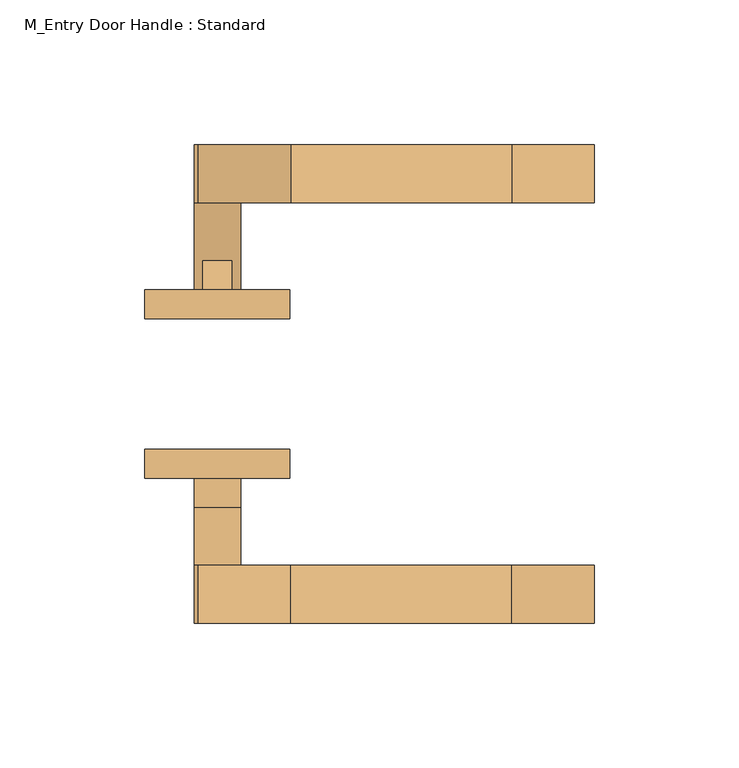
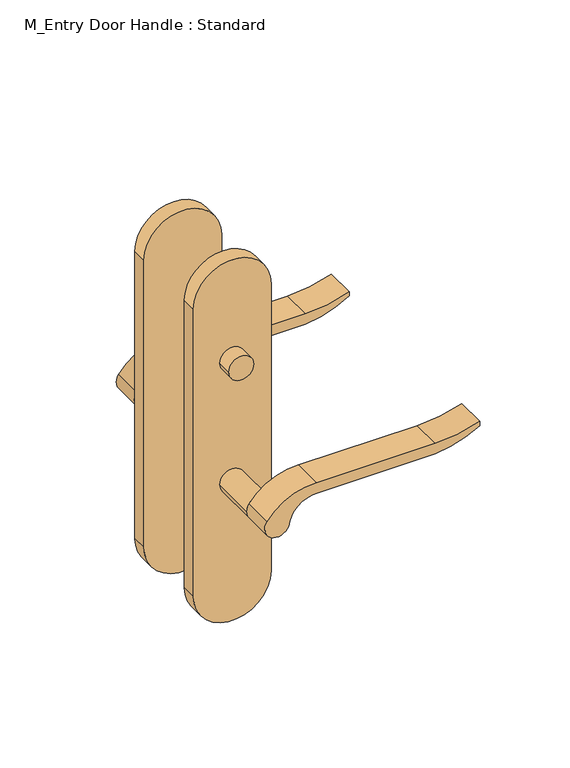
"""IFC4 building model written with IfcOpenShell, lengths in millimetres: door geometry, M_Entry Door Handle : Standard."""

import ifcopenshell
import ifcopenshell.guid

model = None  # the IFC model being written
_history = None  # IfcOwnerHistory: only IFC2X3 demands one
_inside = {}  # id of a spatial element -> (the spatial element, [elements in it])
_under = {}  # id of a project, library or spatial element -> (it, [spatial elements below it])
_declared = {}  # id of a project -> (the project, [libraries it declares])
_typed = {}  # id of a type object -> (the type object, [elements of that type])
_made_of = {}  # id of a material, layer set ... -> (it, [elements and type objects made of it])


def new_model(schema):
    """Start an empty IFC model of exactly this schema.

    Asked for "IFC4X3", IfcOpenShell would pick the latest addendum, in which some entities
    have other attributes; the version numbers below select the first issue.
    IFC2X3 requires an IfcOwnerHistory on every rooted entity: one is made here for all.
    """
    global model, _history
    if schema == "IFC4X3":
        model = ifcopenshell.file(schema_version=(4, 3, 0, 0))
    else:
        model = ifcopenshell.file(schema=schema)
    _inside.clear()
    _under.clear()
    _declared.clear()
    _typed.clear()
    _made_of.clear()
    _history = None
    if model.schema == "IFC2X3":
        org = make("IfcOrganization", Name="unknown")
        user = make(
            "IfcPersonAndOrganization",
            ThePerson=make("IfcPerson", FamilyName="unknown"),
            TheOrganization=org,
        )
        app = make(
            "IfcApplication",
            ApplicationDeveloper=org,
            Version="unknown",
            ApplicationFullName="unknown",
            ApplicationIdentifier="unknown",
        )
        _history = make(
            "IfcOwnerHistory",
            OwningUser=user,
            OwningApplication=app,
            ChangeAction="ADDED",
            CreationDate=0,
        )
    return model


def make(cls, **values):
    """One entity of the class cls with the attributes given. An attribute that is None is left unset."""
    return model.create_entity(
        cls, **{name: value for name, value in values.items() if value is not None}
    )


def rooted(cls, **values):
    """An entity with a GlobalId (a new one), such as an element, a storey or a relation."""
    return make(cls, GlobalId=ifcopenshell.guid.new(), OwnerHistory=_history, **values)


def si_unit(unit_type, name, prefix=None):
    """IfcSIUnit, for example si_unit("LENGTHUNIT", "METRE", prefix="MILLI")."""
    return make("IfcSIUnit", UnitType=unit_type, Prefix=prefix, Name=name)


def assignment(units):
    """IfcUnitAssignment: the units of a project."""
    return None if units is None else make("IfcUnitAssignment", Units=units)


def point(xyz):
    """IfcCartesianPoint."""
    return None if xyz is None else make("IfcCartesianPoint", Coordinates=xyz)


def direction(xyz):
    """IfcDirection."""
    return None if xyz is None else make("IfcDirection", DirectionRatios=xyz)


def frame(location, z_axis=None, x_axis=None):
    """IfcAxis2Placement3D, a coordinate frame: its origin and axes. An axis left out is left unset."""
    return make(
        "IfcAxis2Placement3D",
        Location=point(location),
        Axis=direction(z_axis),
        RefDirection=direction(x_axis),
    )


def frame_2d(location, x_axis=None):
    """IfcAxis2Placement2D, a coordinate frame in the plane: its origin and x axis."""
    return make(
        "IfcAxis2Placement2D", Location=point(location), RefDirection=direction(x_axis)
    )


def origin():
    """The frame at (0, 0, 0) with its axes left unset."""
    return frame((0.0, 0.0, 0.0))


def origin_2d():
    """The frame at (0, 0) in the plane with its x axis left unset."""
    return frame_2d((0.0, 0.0))


def place(relative_to, where):
    """IfcLocalPlacement: puts the frame where relative to a parent placement (None: the world)."""
    return make(
        "IfcLocalPlacement", PlacementRelTo=relative_to, RelativePlacement=where
    )


def context(
    kind, dimensions, precision=None, world=None, true_north=None, identifier=None
):
    """IfcGeometricRepresentationContext, for example the 3D "Model" context."""
    return make(
        "IfcGeometricRepresentationContext",
        ContextIdentifier=identifier,
        ContextType=kind,
        CoordinateSpaceDimension=dimensions,
        Precision=precision,
        WorldCoordinateSystem=world,
        TrueNorth=true_north,
    )


def project(units=None, contexts=None):
    """IfcProject with its units and contexts."""
    return rooted(
        "IfcProject",
        Name="project",
        RepresentationContexts=contexts,
        UnitsInContext=assignment(units),
    )


def spatial(cls, under=None, at=None, **own):
    """A site, building, storey or space (cls), placed at a placement, below another one or the project."""
    s = rooted(cls, ObjectPlacement=at, **own)
    if under is not None:
        _under.setdefault(under.id(), (under, []))[1].append(s)
    return s


def polyline(points):
    """IfcPolyline through the points."""
    return make("IfcPolyline", Points=[point(p) for p in points])


def circle_curve(where, radius):
    """IfcCircle in the frame where."""
    return make("IfcCircle", Position=where, Radius=radius)


def trimmed(basis, trim1, trim2, sense, master):
    """IfcTrimmedCurve: the piece of a basis curve between two trims."""
    return make(
        "IfcTrimmedCurve",
        BasisCurve=basis,
        Trim1=trim1,
        Trim2=trim2,
        SenseAgreement=sense,
        MasterRepresentation=master,
    )


def segment(curve, same_sense, transition):
    """IfcCompositeCurveSegment."""
    return make(
        "IfcCompositeCurveSegment",
        Transition=transition,
        SameSense=same_sense,
        ParentCurve=curve,
    )


def composite_curve(segments, self_intersect=None):
    """IfcCompositeCurve: segments joined end to end."""
    return make("IfcCompositeCurve", Segments=segments, SelfIntersect=self_intersect)


def outline(outer, holes=None, kind="AREA"):
    """IfcArbitraryClosedProfileDef: a profile drawn as a closed curve; with holes, ...WithVoids."""
    if holes is None:
        return make("IfcArbitraryClosedProfileDef", ProfileType=kind, OuterCurve=outer)
    return make(
        "IfcArbitraryProfileDefWithVoids",
        ProfileType=kind,
        OuterCurve=outer,
        InnerCurves=holes,
    )


def extrude(swept, where, along, depth):
    """IfcExtrudedAreaSolid: the profile swept, set in the frame where, extruded along a direction by depth."""
    return make(
        "IfcExtrudedAreaSolid",
        SweptArea=swept,
        Position=where,
        ExtrudedDirection=direction(along),
        Depth=depth,
    )


def shape(context_of_items, identifier, shape_type, items):
    """IfcShapeRepresentation: the items that make up one representation, for example the "Body"."""
    return make(
        "IfcShapeRepresentation",
        ContextOfItems=context_of_items,
        RepresentationIdentifier=identifier,
        RepresentationType=shape_type,
        Items=items,
    )


def source(mapping_origin, context_of_items, identifier, shape_type, items):
    """IfcRepresentationMap: a shape defined once, which mapped items show again and again."""
    return make(
        "IfcRepresentationMap",
        MappingOrigin=mapping_origin,
        MappedRepresentation=shape(context_of_items, identifier, shape_type, items),
    )


def transform(
    local_origin,
    x_axis=None,
    y_axis=None,
    z_axis=None,
    scale=None,
    scale2=None,
    scale3=None,
    uniform=True,
):
    """IfcCartesianTransformationOperator3D, or its non-uniform kind. x_axis, y_axis, z_axis: its Axis1, 2, 3."""
    if uniform:
        return make(
            "IfcCartesianTransformationOperator3D",
            Axis1=direction(x_axis),
            Axis2=direction(y_axis),
            LocalOrigin=point(local_origin),
            Scale=scale,
            Axis3=direction(z_axis),
        )
    return make(
        "IfcCartesianTransformationOperator3DnonUniform",
        Axis1=direction(x_axis),
        Axis2=direction(y_axis),
        LocalOrigin=point(local_origin),
        Scale=scale,
        Axis3=direction(z_axis),
        Scale2=scale2,
        Scale3=scale3,
    )


def mapped(mapping_source, mapping_target):
    """IfcMappedItem: shows the shape of a source again, moved by a transform."""
    return make(
        "IfcMappedItem", MappingSource=mapping_source, MappingTarget=mapping_target
    )


def made_of(thing, what):
    """Note that an element or type object is made of a material, layer set ...; save() writes the relation."""
    if what is not None:
        _made_of.setdefault(what.id(), (what, []))[1].append(thing)
    return thing


def element(
    cls,
    number,
    at=None,
    inside=None,
    cuts=None,
    type_object=None,
    material=None,
    context=None,
    identifier="Body",
    shape_type=None,
    held_by="IfcProductDefinitionShape",
    body=None,
    shapes=None,
    **own,
):
    """One element of the class cls, such as IfcWall. Its Tag is "e" and its number.

    at: its placement. inside: the storey or other place that contains it. cuts: it is an
    opening in that element (IfcRelVoidsElement). A single representation is given by context,
    identifier, shape_type and body (its items); several are given by shapes. held_by: the class
    of the entity that holds the representations. save() writes the other relations.
    """
    e = rooted(cls, Tag="e%d" % number, ObjectPlacement=at, **own)
    if body is not None:
        shapes = [shape(context, identifier, shape_type, body)]
    if shapes is not None:
        e.Representation = make(held_by, Representations=shapes)
    if inside is not None:
        _inside.setdefault(inside.id(), (inside, []))[1].append(e)
    if cuts is not None:
        rooted(
            "IfcRelVoidsElement", RelatingBuildingElement=cuts, RelatedOpeningElement=e
        )
    if type_object is not None:
        _typed.setdefault(type_object.id(), (type_object, []))[1].append(e)
    return made_of(e, material)


def aggregate(whole, parts):
    """IfcRelAggregates: a whole, such as a stair, and the parts it consists of."""
    return rooted("IfcRelAggregates", RelatingObject=whole, RelatedObjects=parts)


def save(model, path):
    """Write the relations noted so far, then the file.

    IfcRelAggregates (storeys below a building ...), IfcRelContainedInSpatialStructure (elements
    in a storey), IfcRelDefinesByType, IfcRelAssociatesMaterial and IfcRelDeclares: one each for
    every whole, place, type object, material and project.
    """
    for whole, parts in _under.values():
        aggregate(whole, parts)
    for where, things in _inside.values():
        rooted(
            "IfcRelContainedInSpatialStructure",
            RelatedElements=things,
            RelatingStructure=where,
        )
    for kind, things in _typed.values():
        rooted("IfcRelDefinesByType", RelatedObjects=things, RelatingType=kind)
    for what, things in _made_of.values():
        rooted("IfcRelAssociatesMaterial", RelatedObjects=things, RelatingMaterial=what)
    for by, libraries in _declared.values():
        rooted("IfcRelDeclares", RelatingContext=by, RelatedDefinitions=libraries)
    model.write(path)


def m_entry_door_handle_standard_7ac350b3(model_context):
    return source(origin(), model_context, "Body", "SweptSolid", [
        extrude(outline(polyline([(-5.0, 42.5), (5.0, 42.5), (5.0, 32.5), (-5.0, 32.5), (-5.0, 42.5)])), frame((0.0, 0.0, 67.5), z_axis=(0.0, 0.0, 1.0), x_axis=(1.0, 0.0, 0.0)), (0.0, 0.0, 1.0), 30.0),
        extrude(outline(composite_curve([segment(trimmed(circle_curve(frame_2d((82.5, 0.0)), 8.0), [point((82.5, 8.0))], [point((82.5, -8.0))], False, "CARTESIAN"), True, "CONTINUOUS"), segment(trimmed(circle_curve(frame_2d((82.5, 0.0)), 8.0), [point((82.5, -8.0))], [point((82.5, 8.0))], False, "CARTESIAN"), True, "CONTINUOUS")], self_intersect=False)), frame((0.0, -42.5, 0.0), z_axis=(0.0, 1.0, 0.0), x_axis=(0.0, 0.0, 1.0)), (0.0, 0.0, 1.0), 10.0),
        extrude(outline(composite_curve([segment(trimmed(circle_curve(origin_2d(), 8.0), [point((4.6523287, -6.5081363))], [point((0.0, 8.0))], False, "CARTESIAN"), True, "CONTINUOUS"), segment(trimmed(circle_curve(frame_2d((-5.1261387, 25.3861901)), 18.1261387), [point((0.0, 8.0))], [point((13.0, 25.3861901))], True, "CARTESIAN"), True, "CONTINUOUS"), segment(polyline([(13.0, 25.3861901), (13.0, 101.6435909)]), True, "CONTINUOUS"), segment(trimmed(circle_curve(frame_2d((72.2709207, 98.0603388)), 59.3791355), [point((13.0, 101.6435909))], [point((22.2135558, 130.0))], False, "CARTESIAN"), True, "CONTINUOUS"), segment(polyline([(22.2135558, 130.0), (25.0, 130.0)]), True, "CONTINUOUS"), segment(trimmed(circle_curve(frame_2d((103.2850638, 101.5772091)), 83.2850902), [point((25.0, 130.0))], [point((20.0, 101.6435909))], True, "CARTESIAN"), True, "CONTINUOUS"), segment(polyline([(20.0, 101.6435909), (20.0, 25.3674333)]), True, "CONTINUOUS"), segment(trimmed(circle_curve(frame_2d((-17.2444479, 23.6675129)), 37.2832219), [point((20.0, 25.3674333))], [point((4.6523287, -6.5081363))], False, "CARTESIAN"), True, "CONTINUOUS")], self_intersect=False)), frame((0.0, 62.5, 0.0), z_axis=(0.0, 1.0, 0.0), x_axis=(0.0, 0.0, 1.0)), (0.0, 0.0, 1.0), 20.0),
        extrude(outline(composite_curve([segment(trimmed(circle_curve(frame_2d((-5.1261318, 25.3861878)), 18.1261318), [point((-9.7e-06, 8.0))], [point((13.0, 25.3861878))], True, "CARTESIAN"), True, "CONTINUOUS"), segment(polyline([(13.0, 25.3861878), (13.0, 101.6435909)]), True, "CONTINUOUS"), segment(trimmed(circle_curve(frame_2d((72.2709207, 98.0603388)), 59.3791355), [point((13.0, 101.6435909))], [point((22.2135558, 130.0))], False, "CARTESIAN"), True, "CONTINUOUS"), segment(polyline([(22.2135558, 130.0), (25.0, 130.0)]), True, "CONTINUOUS"), segment(trimmed(circle_curve(frame_2d((103.2850638, 101.5772091)), 83.2850902), [point((25.0, 130.0))], [point((20.0, 101.6435909))], True, "CARTESIAN"), True, "CONTINUOUS"), segment(polyline([(20.0, 101.6435909), (20.0, 25.3674333)]), True, "CONTINUOUS"), segment(trimmed(circle_curve(frame_2d((-17.2444479, 23.6675129)), 37.2832219), [point((20.0, 25.3674333))], [point((4.6523287, -6.5081363))], False, "CARTESIAN"), True, "CONTINUOUS"), segment(trimmed(circle_curve(origin_2d(), 8.0), [point((4.6523287, -6.5081363))], [point((-9.7e-06, 8.0))], False, "CARTESIAN"), True, "CONTINUOUS")], self_intersect=False)), frame((0.0, -82.5, 0.0), z_axis=(0.0, 1.0, 0.0), x_axis=(0.0, 0.0, 1.0)), (0.0, 0.0, 1.0), 20.0),
        extrude(outline(composite_curve([segment(trimmed(circle_curve(origin_2d(), 8.0), [point((0.0, 8.0))], [point((0.0, -8.0))], False, "CARTESIAN"), True, "CONTINUOUS"), segment(trimmed(circle_curve(origin_2d(), 8.0), [point((0.0, -8.0))], [point((0.0, 8.0))], False, "CARTESIAN"), True, "CONTINUOUS")], self_intersect=False)), frame((0.0, 32.5, 0.0), z_axis=(0.0, 1.0, 0.0), x_axis=(0.0, 0.0, 1.0)), (0.0, 0.0, 1.0), 30.0),
        extrude(outline(composite_curve([segment(trimmed(circle_curve(origin_2d(), 8.0), [point((0.0, 8.0))], [point((0.0, -8.0))], False, "CARTESIAN"), True, "CONTINUOUS"), segment(trimmed(circle_curve(origin_2d(), 8.0), [point((0.0, -8.0))], [point((0.0, 8.0))], False, "CARTESIAN"), True, "CONTINUOUS")], self_intersect=False)), frame((0.0, -62.5, 0.0), z_axis=(0.0, 1.0, 0.0), x_axis=(0.0, 0.0, 1.0)), (0.0, 0.0, 1.0), 30.0),
        extrude(outline(composite_curve([segment(trimmed(circle_curve(frame_2d((-70.0, 0.0)), 25.0), [point((-70.0, -25.0))], [point((-70.0, 25.0))], False, "CARTESIAN"), True, "CONTINUOUS"), segment(polyline([(-70.0, 25.0), (125.0, 25.0)]), True, "CONTINUOUS"), segment(trimmed(circle_curve(frame_2d((125.0, 0.0)), 25.0), [point((125.0, 25.0))], [point((125.0, -25.0))], False, "CARTESIAN"), True, "CONTINUOUS"), segment(polyline([(125.0, -25.0), (-70.0, -25.0)]), True, "CONTINUOUS")], self_intersect=False)), frame((0.0, 22.5, 0.0), z_axis=(0.0, 1.0, 0.0), x_axis=(0.0, 0.0, 1.0)), (0.0, 0.0, 1.0), 10.0),
        extrude(outline(composite_curve([segment(trimmed(circle_curve(frame_2d((-70.0, 0.0)), 25.0), [point((-70.0, -25.0))], [point((-70.0, 25.0))], False, "CARTESIAN"), True, "CONTINUOUS"), segment(polyline([(-70.0, 25.0), (125.0, 25.0)]), True, "CONTINUOUS"), segment(trimmed(circle_curve(frame_2d((125.0, 0.0)), 25.0), [point((125.0, 25.0))], [point((125.0, -25.0))], False, "CARTESIAN"), True, "CONTINUOUS"), segment(polyline([(125.0, -25.0), (-70.0, -25.0)]), True, "CONTINUOUS")], self_intersect=False)), frame((0.0, -32.5, 0.0), z_axis=(0.0, 1.0, 0.0), x_axis=(0.0, 0.0, 1.0)), (0.0, 0.0, 1.0), 10.0),
    ])


if __name__ == "__main__":
    model = new_model("IFC4")
    model_context = context("Model", 3, world=origin())
    ifc_project = project(units=[si_unit("LENGTHUNIT", "METRE", prefix="MILLI")], contexts=[model_context])
    site = spatial("IfcSite", under=ifc_project)
    building = spatial("IfcBuilding", under=site)
    placement = place(None, origin())
    m_entry_door_handle_standard_shape = m_entry_door_handle_standard_7ac350b3(model_context)
    element("IfcDoor", 1, ObjectType="M_Entry Door Handle : Standard", at=placement, inside=building, context=model_context, shape_type="MappedRepresentation", body=[
        mapped(m_entry_door_handle_standard_shape, transform((0.0, 0.0, 0.0), x_axis=(1.0, 0.0, 0.0), y_axis=(0.0, 1.0, 0.0), z_axis=(0.0, 0.0, 1.0))),
    ])
    save(model, "model.ifc")

# Revit data of these elements
# Type "M_Entry Door Handle : Standard"
#   Type Mark = "50"
#   Analytic Construction = "<None>"
#   Thickness = 4.5 cm
#   Handle Material = Aluminum
#   Function = (empty or 0)
#   Construction Type = (empty or 0)
# Element 1 (IfcDoor, "M_Entry Door Handle : Standard")
#   Materials on its faces: "Aluminum"
# Materials
#   "Aluminum": class "Metal", colour RGB 247 247 247, transparency 0, Description = "Aluminum 6061", Cost = 0
